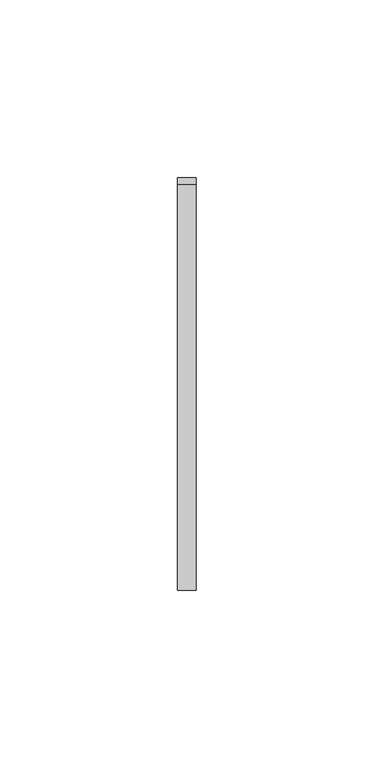
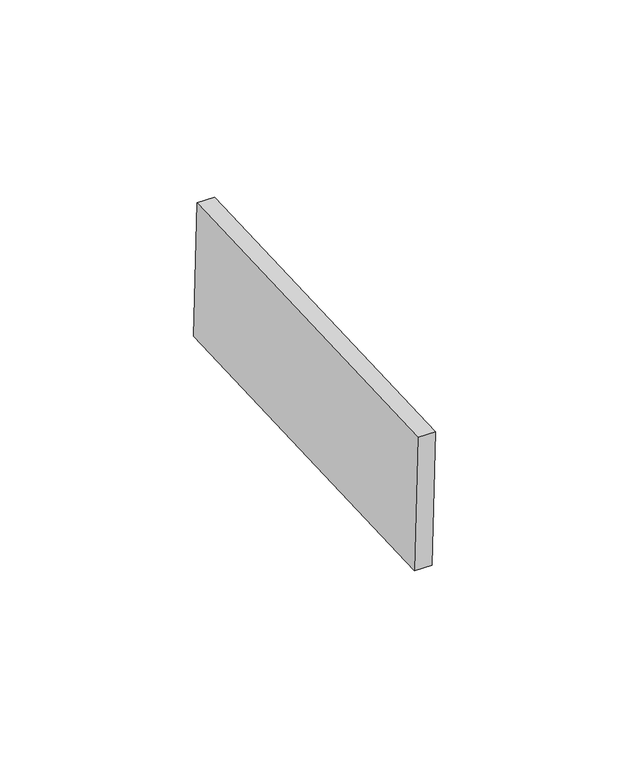
"""IFC4 building model written with IfcOpenShell, lengths in millimetres: proxy geometry, Inner panel:Inner panel:1:Inner panel:1 : Inner panel:Inner panel:300324:2:Inner panel:1:Inner panel:1 : Inner panel:Inner panel:300324:2 : Inner panel:Inner panel:1:Inner panel:1 : Inner panel:Inner panel:300324:300043:87 : Inner panel:Inner panel:1:Inner panel:1 : Inner panel:Inner panel:300324:2:Inner panel:1:Inner panel:1 : Inner panel:Inner panel:300324:2 : Inner panel:Inner panel:1:Inner panel:1 : Inner panel:Inner panel:300324:300043:308120."""

from ifc_helpers import new_model, si_unit, frame, origin, place, context, project, spatial, polyline, outline, extrude, source, transform, mapped, element, save


def generic_models_01e034dc(model_context):
    return source(origin(), model_context, "Body", "SweptSolid", [
        extrude(outline(polyline([(0.0, -114.2999999), (0.0, 0.0), (5.2138089, 0.0), (5.2138089, -114.2999999), (0.0, -114.2999999)])), frame((591904.595117, -576618.8219505, 4051.6214343), z_axis=(0.0, -0.04163054471216399, 0.9991330730923527), x_axis=(-1.0, 0.0, 0.0)), (0.0, 0.0, 1.0), 43.2233908),
    ])


if __name__ == "__main__":
    model = new_model("IFC4")
    model_context = context("Model", 3, world=origin())
    ifc_project = project(units=[si_unit("LENGTHUNIT", "METRE", prefix="MILLI")], contexts=[model_context])
    site = spatial("IfcSite", under=ifc_project)
    building = spatial("IfcBuilding", under=site)
    placement = place(None, origin())
    generic_models_shape = generic_models_01e034dc(model_context)
    element("IfcBuildingElementProxy", 1, Name="Inner panel:Inner panel:1:Inner panel:1 : Inner panel:Inner panel:300324:2:Inner panel:1:Inner panel:1 : Inner panel:Inner panel:300324:2 : Inner panel:Inner panel:1:Inner panel:1 : Inner panel:Inner panel:300324:300043:87 : Inner panel:Inner panel:1:Inner panel:1 : Inner panel:Inner panel:300324:2:Inner panel:1:Inner panel:1 : Inner panel:Inner panel:300324:2 : Inner panel:Inner panel:1:Inner panel:1 : Inner panel:Inner panel:300324:300043:308120", ObjectType="Inner panel:Inner panel:1:Inner panel:1 : Inner panel:Inner panel:300324:2:Inner panel:1:Inner panel:1 : Inner panel:Inner panel:300324:2 : Inner panel:Inner panel:1:Inner panel:1 : Inner panel:Inner panel:300324:300043:87 : Inner panel:Inner panel:1:Inner panel:1 : Inner panel:Inner panel:300324:2:Inner panel:1:Inner panel:1 : Inner panel:Inner panel:300324:2 : Inner panel:Inner panel:1:Inner panel:1 : Inner panel:Inner panel:300324:300043:308120", at=placement, inside=building, context=model_context, shape_type="MappedRepresentation", body=[
        mapped(generic_models_shape, transform((0.0, 0.0, 0.0), x_axis=(1.0, 0.0, 0.0), y_axis=(0.0, 1.0, 0.0), z_axis=(0.0, 0.0, 1.0))),
    ])
    save(model, "model.ifc")

# Revit data of these elements
# Type "Inner panel:Inner panel:1:Inner panel:1 : Inner panel:Inner panel:300324:2:Inner panel:1:Inner panel:1 : Inner panel:Inner panel:300324:2 : Inner panel:Inner panel:1:Inner panel:1 : Inner panel:Inner panel:300324:300043:87 : Inner panel:Inner panel:1:Inner panel:1 : Inner panel:Inner panel:300324:2:Inner panel:1:Inner panel:1 : Inner panel:Inner panel:300324:2 : Inner panel:Inner panel:1:Inner panel:1 : Inner panel:Inner panel:300324:300043:308120"
#   NameOverride = "Inner panel:Inner panel:1:Inner panel:1 : Inner panel:Inner panel:300324:2:Inner panel:1:Inner panel:1 : Inner panel:Inner panel:300324:2 : Inner panel:Inner panel:1:Inner panel:1 : Inner panel:Inner panel:300324:300043:308120"
#   ObjectTypeOverride = "Inner panel:1:Inner panel:1 : Inner panel:Inner panel:300324:2 : Inner panel:Inner panel:1:Inner panel:1 : Inner panel:Inner panel:300324:300043"
#   Reference = "Inner panel"
#   Tag = "308120"
# Element 1 (IfcBuildingElementProxy, "Inner panel:Inner panel:1:Inner panel:1 : Inner panel:Inner panel:300324:2:Inner panel:1:Inner panel:1 : Inner panel:Inner panel:300324:2 : Inner panel:Inner panel:1:Inner panel:1 : Inner panel:Inner panel:300324:300043:87 : Inner panel:Inner panel:1:Inner panel:1 : Inner panel:Inner panel:300324:2:Inner panel:1:Inner panel:1 : Inner panel:Inner panel:300324:2 : Inner panel:Inner panel:1:Inner panel:1 : Inner panel:Inner panel:300324:300043:308120")
#   Materials on its faces: "SLIDING CLIP"
# Materials
#   "SLIDING CLIP": class "Generic", colour RGB 120 120 120, transparency 0, Cost = 0
